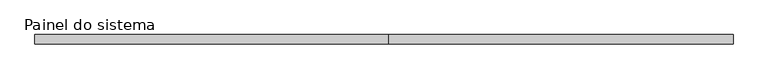
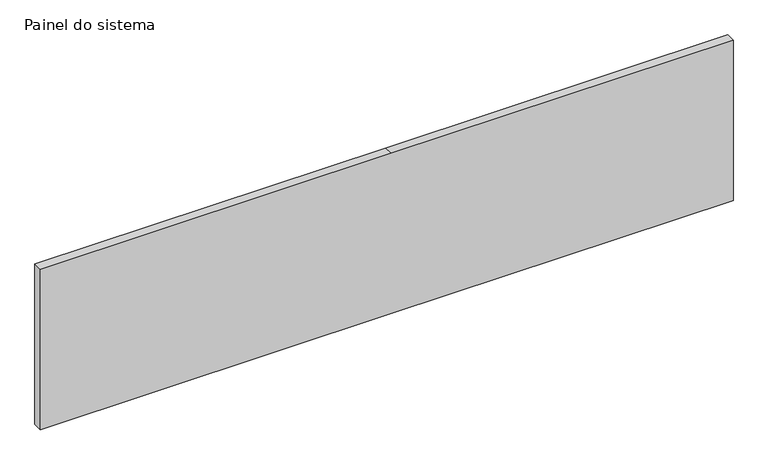
"""IFC4 building model written with IfcOpenShell, lengths in millimetres: plate geometry, Painel do sistema : Envidraçado."""

from ifc_helpers import new_model, si_unit, frame, origin, place, context, project, spatial, polyline, outline, extrude, source, transform, mapped, element, save


def painel_do_sistema_33a988d1(model_context):
    return source(origin(), model_context, "Body", "SweptSolid", [
        extrude(outline(polyline([(0.0, -918.5166667), (0.0, 12.4999998), (0.0, 918.5166667), (450.0, 918.5166667), (450.0, 12.4999998), (450.0, -918.5166667), (0.0, -918.5166667)])), frame((0.0, 24.5, 0.0), z_axis=(0.0, 1.0, 0.0), x_axis=(0.0, 0.0, 1.0)), (0.0, 0.0, 1.0), 25.0),
    ])


if __name__ == "__main__":
    model = new_model("IFC4")
    model_context = context("Model", 3, world=origin())
    ifc_project = project(units=[si_unit("LENGTHUNIT", "METRE", prefix="MILLI")], contexts=[model_context])
    site = spatial("IfcSite", under=ifc_project)
    building = spatial("IfcBuilding", under=site)
    placement = place(None, origin())
    painel_do_sistema_shape = painel_do_sistema_33a988d1(model_context)
    element("IfcPlate", 1, ObjectType="Painel do sistema : Envidraçado", at=placement, inside=building, context=model_context, shape_type="MappedRepresentation", body=[
        mapped(painel_do_sistema_shape, transform((0.0, 0.0, 0.0), x_axis=(1.0, 0.0, 0.0), y_axis=(0.0, 1.0, 0.0), z_axis=(0.0, 0.0, 1.0))),
    ])
    save(model, "model.ifc")

# Revit data of these elements
# Type "Painel do sistema : Envidraçado"
#   Construction Type Id = "GSP4R"
#   Analytic Construction = "Vidraça única Pilkington 1/8 pol"
#   Visual Light Transmittance = 0.9
#   Solar Heat Gain Coefficient = 0.86
#   Heat Transfer Coefficient (U) = 6.7069 W/(m²·K)
# Element 1 (IfcPlate, "Painel do sistema : Envidraçado")
#   Materials on its faces: ".VIDRO GENÉRICO"
# Materials
#   ".VIDRO GENÉRICO": class ".CC_VIDRO", colour RGB 0 128 192, transparency 0.9, Description = "Vidro comum", Cost = 0
